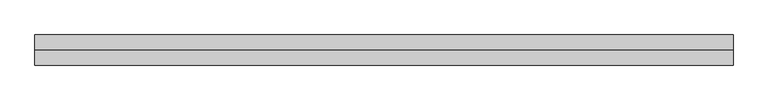
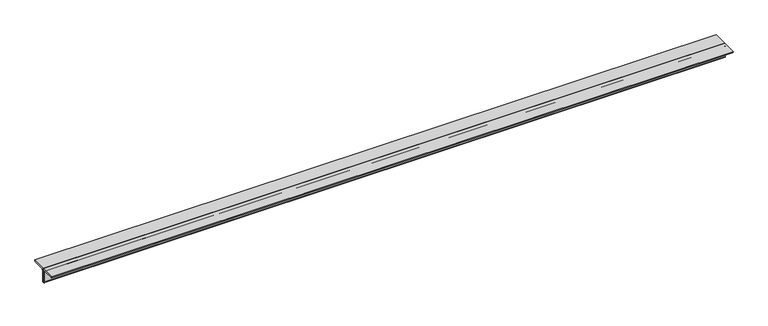
"""IFC4 building model written with IfcOpenShell, lengths in millimetres: member geometry, Steel Framing_2Ls_KS : H_SB_AR_S02_2Ls-100x100x10_VBR1."""

from ifc_helpers import new_model, si_unit, point, frame, frame_2d, origin, place, context, project, spatial, polyline, circle_curve, trimmed, segment, composite_curve, outline, extrude, source, transform, mapped, element, save


def member_1a99136a(model_context):
    return source(origin(), model_context, "Body", "SweptSolid", [
        extrude(outline(composite_curve([segment(polyline([(0.0, 28.2), (100.0, 28.2)]), True, "CONTINUOUS"), segment(trimmed(circle_curve(frame_2d((90.0, 28.2)), 10.0), [point((100.0, 28.2))], [point((90.0, 18.2))], False, "CARTESIAN"), True, "CONTINUOUS"), segment(polyline([(90.0, 18.2), (20.0, 18.2)]), True, "CONTINUOUS"), segment(trimmed(circle_curve(frame_2d((20.0, 8.2)), 10.0), [point((20.0, 18.2))], [point((10.0, 8.2))], True, "CARTESIAN"), True, "CONTINUOUS"), segment(polyline([(10.0, 8.2), (10.0, -61.8)]), True, "CONTINUOUS"), segment(trimmed(circle_curve(frame_2d((0.0, -61.8)), 10.0), [point((10.0, -61.8))], [point((0.0, -71.8))], False, "CARTESIAN"), True, "CONTINUOUS"), segment(polyline([(0.0, -71.8), (0.0, 28.2)]), True, "CONTINUOUS")], self_intersect=False)), frame((-2442.577408, 0.0, 0.0), z_axis=(1.0, 0.0, 0.0), x_axis=(0.0, 1.0, 0.0)), (0.0, 0.0, 1.0), 4633.0171831),
        extrude(outline(composite_curve([segment(polyline([(0.0, 28.2), (0.0, -71.8)]), True, "CONTINUOUS"), segment(trimmed(circle_curve(frame_2d((0.0, -61.8)), 10.0), [point((0.0, -71.8))], [point((-10.0, -61.8))], False, "CARTESIAN"), True, "CONTINUOUS"), segment(polyline([(-10.0, -61.8), (-10.0, 8.2)]), True, "CONTINUOUS"), segment(trimmed(circle_curve(frame_2d((-20.0, 8.2)), 10.0), [point((-10.0, 8.2))], [point((-20.0, 18.2))], True, "CARTESIAN"), True, "CONTINUOUS"), segment(polyline([(-20.0, 18.2), (-90.0, 18.2)]), True, "CONTINUOUS"), segment(trimmed(circle_curve(frame_2d((-90.0, 28.2)), 10.0), [point((-90.0, 18.2))], [point((-100.0, 28.2))], False, "CARTESIAN"), True, "CONTINUOUS"), segment(polyline([(-100.0, 28.2), (0.0, 28.2)]), True, "CONTINUOUS")], self_intersect=False)), frame((-2442.577408, 0.0, 0.0), z_axis=(1.0, 0.0, 0.0), x_axis=(0.0, 1.0, 0.0)), (0.0, 0.0, 1.0), 4633.0171831),
    ])


if __name__ == "__main__":
    model = new_model("IFC4")
    model_context = context("Model", 3, world=origin())
    ifc_project = project(units=[si_unit("LENGTHUNIT", "METRE", prefix="MILLI")], contexts=[model_context])
    site = spatial("IfcSite", under=ifc_project)
    building = spatial("IfcBuilding", under=site)
    placement = place(None, origin())
    member_shape = member_1a99136a(model_context)
    element("IfcMember", 1, ObjectType="Steel Framing_2Ls_KS : H_SB_AR_S02_2Ls-100x100x10_VBR1", at=placement, inside=building, context=model_context, shape_type="MappedRepresentation", body=[
        mapped(member_shape, transform((0.0, 0.0, 0.0), x_axis=(1.0, 0.0, 0.0), y_axis=(0.0, 1.0, 0.0), z_axis=(0.0, 0.0, 1.0))),
    ])
    save(model, "model.ifc")

# Revit data of these elements
# Type "Steel Framing_2Ls_KS : H_SB_AR_S02_2Ls-100x100x10_VBR1"
#   Type Comments = "MAIN"
#   Type Mark = "VBR1"
#   H_SectionID = "2Ls-100x100x10"
#   Assembly Code = "B10"
#   Legs = "LLBB"
#   H_Ratio for Additional Steel Plate = 0.2
#   W = 0
#   Perimeter = 0.80 m²/m
#   Nominal Weight = 29.80 kgf/m
#   Length [instance default] = 1524 mm
#   Space = 0 mm
#   b = 100 mm
#   d = 100 mm
#   t = 10 mm
#   y = 28.2 mm
#   A = 0.0038 m²
#   Structural Material [instance default] = Steel, 45-345
# Element 1 (IfcMember, "Steel Framing_2Ls_KS : H_SB_AR_S02_2Ls-100x100x10_VBR1")
#   Materials on its faces: "Steel, 45-345"
# Materials
#   "Steel, 45-345": class "Metal", colour RGB 189 187 185, transparency 0, Description = "Steel 345 MPa", Cost = 0
